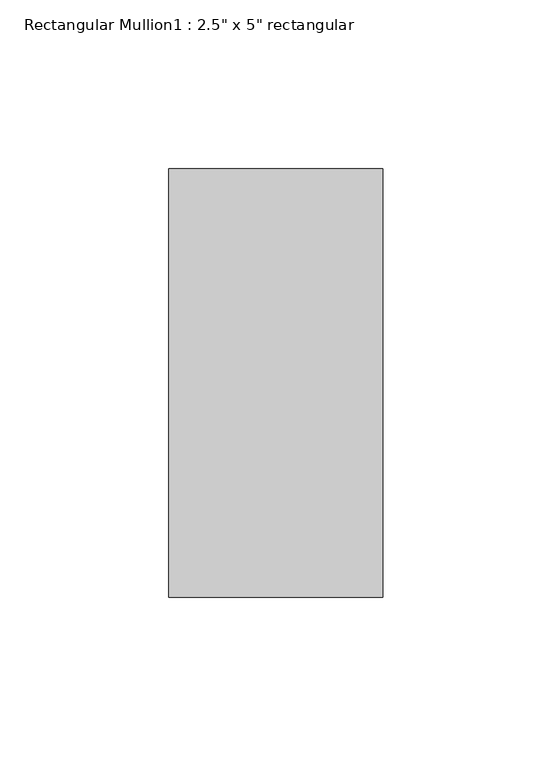
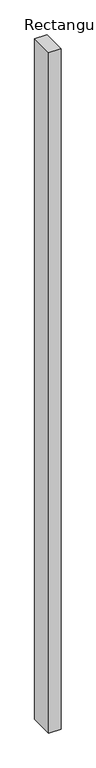
"""IFC4 building model written with IfcOpenShell, lengths in millimetres: member geometry."""

from ifc_helpers import new_model, si_unit, frame, origin, place, context, project, spatial, polyline, outline, extrude, source, transform, mapped, element, save


def member_bbf28ac8(model_context):
    return source(origin(), model_context, "Body", "SweptSolid", [
        extrude(outline(polyline([(0.0, 63.5), (0.0, -63.5), (-63.5, -63.5), (-63.5, 63.5), (0.0, 63.5)])), frame((0.0, 0.0, -3746.5), z_axis=(0.0, 0.0, 1.0), x_axis=(1.0, 0.0, 0.0)), (0.0, 0.0, 1.0), 3746.5),
    ])


if __name__ == "__main__":
    model = new_model("IFC4")
    model_context = context("Model", 3, world=origin())
    ifc_project = project(units=[si_unit("LENGTHUNIT", "METRE", prefix="MILLI")], contexts=[model_context])
    site = spatial("IfcSite", under=ifc_project)
    building = spatial("IfcBuilding", under=site)
    placement = place(None, origin())
    member_shape = member_bbf28ac8(model_context)
    element("IfcMember", 1, ObjectType="Rectangular Mullion1 : 2.5\" x 5\" rectangular", at=placement, inside=building, context=model_context, shape_type="MappedRepresentation", body=[
        mapped(member_shape, transform((0.0, 0.0, 0.0), x_axis=(1.0, 0.0, 0.0), y_axis=(0.0, 1.0, 0.0), z_axis=(0.0, 0.0, 1.0))),
    ])
    save(model, "model.ifc")

# Revit data of these elements
# Type "Rectangular Mullion1 : 2.5\" x 5\" rectangular"
#   built-in parameter 1007304 = 0.416667 (stored number, unit not read)
#   built-in parameter 1007301 = 0.104167 (stored number, unit not read)
#   built-in parameter 1007300 = 0.104167 (stored number, unit not read)
# Element 1 (IfcMember, "Rectangular Mullion1 : 2.5\" x 5\" rectangular")
#   Materials on its faces: "support-frame"
# Materials
#   "support-frame": class "Unassigned", colour RGB 233 233 233, transparency 0, Cost = 0
